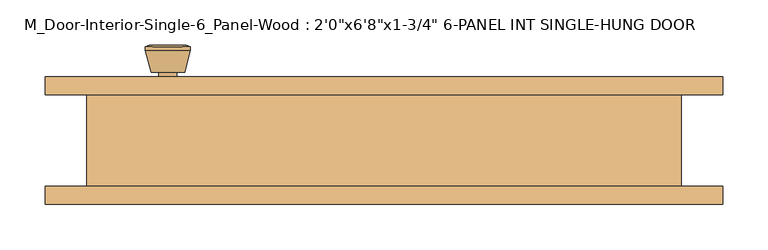
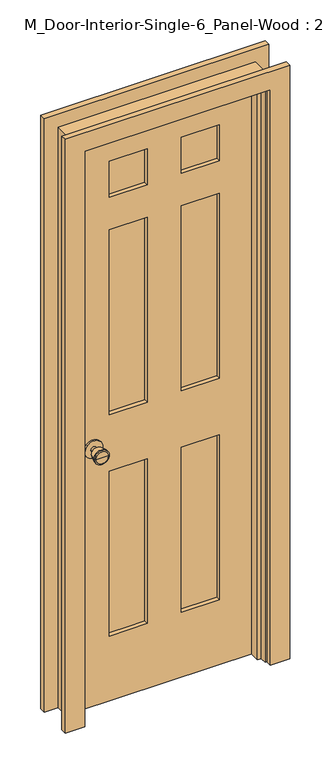
"""IFC4 building model written with IfcOpenShell, lengths in millimetres: door geometry."""

from ifc_helpers import new_model, si_unit, point, frame, frame_2d, origin, place, context, project, spatial, polyline, circle_curve, trimmed, segment, composite_curve, outline, extrude, faceted_brep, source, transform, mapped, element, save
from ifc_brep_helpers import plane_surface, cylinder_surface, revolved_surface, advanced_brep


def door_8ef89e6c(model_context):
    return source(origin(), model_context, "Body", "SolidModel", [
        advanced_brep(
        [(-239.8, -2.825, 914.4), (-229.8, -2.825, 914.4), (-249.8, -2.825, 914.4), (-219.3241324, -51.825, 914.4), (-239.8, -51.825, 914.4), (-260.2758676, -51.825, 914.4), (-214.8, -49.9971319, 914.4), (-264.8, -49.9971319, 914.4), (-214.8, -46.5334537, 914.4), (-264.8, -46.5334537, 914.4), (-221.163764, -21.825, 914.4), (-258.436236, -21.825, 914.4), (-229.8, -21.825, 914.4), (-249.8, -21.825, 914.4)],
        [
            (0, 1),
            (1, 2, circle_curve(frame((-239.8, -2.825, 914.4), z_axis=(0.0, 1.0, 0.0), x_axis=(-1.0, 0.0, 0.0)), 10.0)),
            (2, 0),
            (2, 1, circle_curve(frame((-239.8, -2.825, 914.4), z_axis=(0.0, 1.0, 0.0), x_axis=(-1.0, 0.0, 0.0)), 10.0)),
            (3, 4),
            (4, 5),
            (5, 3, circle_curve(frame((-239.8, -51.825, 914.4), z_axis=(0.0, -1.0, 0.0), x_axis=(-1.0, 0.0, 0.0)), 20.4758676)),
            (3, 5, circle_curve(frame((-239.8, -51.825, 914.4), z_axis=(0.0, -1.0, 0.0), x_axis=(-1.0, 0.0, 0.0)), 20.4758676)),
            (6, 3),
            (5, 7),
            (7, 6, circle_curve(frame((-239.8, -49.9971319, 914.4), z_axis=(0.0, -1.0, 0.0), x_axis=(-1.0, 0.0, 0.0)), 25.0)),
            (6, 7, circle_curve(frame((-239.8, -49.9971319, 914.4), z_axis=(0.0, -1.0, 0.0), x_axis=(-1.0, 0.0, 0.0)), 25.0)),
            (8, 6),
            (7, 9),
            (9, 8, circle_curve(frame((-239.8, -46.5334537, 914.4), z_axis=(0.0, -1.0, 0.0), x_axis=(-1.0, 0.0, 0.0)), 25.0)),
            (8, 9, circle_curve(frame((-239.8, -46.5334537, 914.4), z_axis=(0.0, -1.0, 0.0), x_axis=(-1.0, 0.0, 0.0)), 25.0)),
            (10, 8),
            (9, 11),
            (11, 10, circle_curve(frame((-239.8, -21.825, 914.4), z_axis=(0.0, -1.0, 0.0), x_axis=(-1.0, 0.0, 0.0)), 18.636236)),
            (10, 11, circle_curve(frame((-239.8, -21.825, 914.4), z_axis=(0.0, -1.0, 0.0), x_axis=(-1.0, 0.0, 0.0)), 18.636236)),
            (12, 10),
            (11, 13),
            (13, 12, circle_curve(frame((-239.8, -21.825, 914.4), z_axis=(0.0, -1.0, 0.0), x_axis=(-1.0, 0.0, 0.0)), 10.0)),
            (12, 13, circle_curve(frame((-239.8, -21.825, 914.4), z_axis=(0.0, -1.0, 0.0), x_axis=(-1.0, 0.0, 0.0)), 10.0)),
            (1, 12),
            (13, 2),
        ],
        [
            plane_surface(frame((-239.8, -2.825, 914.4), z_axis=(0.0, 1.0, 0.0), x_axis=(-1.0, 0.0, 0.0))),
            plane_surface(frame((-239.8, -51.825, 914.4), z_axis=(0.0, -1.0, 0.0), x_axis=(-1.0, 0.0, 0.0))),
            revolved_surface(polyline([(-260.2758676, -51.825, 914.4), (-264.8, -49.9971319, 914.4)]), (-239.8, -2.825, 914.4), (0.0, 1.0, 0.0)),
            cylinder_surface(frame((-239.8, -2.825, 914.4), z_axis=(0.0, 1.0, 0.0), x_axis=(-1.0, 0.0, 0.0)), 25.0),
            revolved_surface(polyline([(-264.8, -46.5334537, 914.4), (-258.436236, -21.825, 914.4)]), (-239.8, -2.825, 914.4), (0.0, 1.0, 0.0)),
            plane_surface(frame((-239.8, -21.825, 914.4), z_axis=(0.0, 1.0, 0.0), x_axis=(-1.0, 0.0, 0.0))),
            cylinder_surface(frame((-239.8, -2.825, 914.4), z_axis=(0.0, 1.0, 0.0), x_axis=(-1.0, 0.0, 0.0)), 10.0),
        ],
        [
            (0, [[1, 2, 3]]),
            (0, [[-3, 4, -1]]),
            (1, [[5, 6, 7]]),
            (1, [[-6, -5, 8]]),
            (2, [[9, -7, 10, 11]]),
            (2, [[-10, -8, -9, 12]]),
            (3, [[13, -11, 14, 15]]),
            (3, [[-14, -12, -13, 16]]),
            (4, [[17, -15, 18, 19]]),
            (4, [[-18, -16, -17, 20]]),
            (5, [[21, -19, 22, 23]]),
            (5, [[-22, -20, -21, 24]]),
            (6, [[25, -23, 26, -2]]),
            (6, [[-26, -24, -25, -4]]),
        ],
    ),
        extrude(outline(composite_curve([segment(trimmed(circle_curve(frame_2d((914.4, -239.8)), 30.0), [point((914.4, -269.8))], [point((914.4, -209.8))], False, "CARTESIAN"), True, "CONTINUOUS"), segment(trimmed(circle_curve(frame_2d((914.4, -239.8)), 30.0), [point((914.4, -209.8))], [point((914.4, -269.8))], False, "CARTESIAN"), True, "CONTINUOUS")], self_intersect=False)), frame((0.0, -2.825, 0.0), z_axis=(0.0, 1.0, 0.0), x_axis=(0.0, 0.0, 1.0)), (0.0, 0.0, 1.0), 6.0),
        advanced_brep(
        [(-239.8, 53.625, 914.4), (-249.8, 53.625, 914.4), (-229.8, 53.625, 914.4), (-219.3241324, 102.625, 914.4), (-260.2758676, 102.625, 914.4), (-239.8, 102.625, 914.4), (-214.8, 100.7971319, 914.4), (-264.8, 100.7971319, 914.4), (-214.8, 97.3334537, 914.4), (-264.8, 97.3334537, 914.4), (-221.163764, 72.625, 914.4), (-258.436236, 72.625, 914.4), (-229.8, 72.625, 914.4), (-249.8, 72.625, 914.4)],
        [
            (0, 1),
            (1, 2, circle_curve(frame((-239.8, 53.625, 914.4), z_axis=(0.0, -1.0, 0.0), x_axis=(-1.0, 0.0, 0.0)), 10.0)),
            (2, 0),
            (2, 1, circle_curve(frame((-239.8, 53.625, 914.4), z_axis=(0.0, -1.0, 0.0), x_axis=(-1.0, 0.0, 0.0)), 10.0)),
            (3, 4, circle_curve(frame((-239.8, 102.625, 914.4), z_axis=(0.0, 1.0, 0.0), x_axis=(-1.0, 0.0, 0.0)), 20.4758676)),
            (4, 5),
            (5, 3),
            (4, 3, circle_curve(frame((-239.8, 102.625, 914.4), z_axis=(0.0, 1.0, 0.0), x_axis=(-1.0, 0.0, 0.0)), 20.4758676)),
            (6, 7, circle_curve(frame((-239.8, 100.7971319, 914.4), z_axis=(0.0, 1.0, 0.0), x_axis=(-1.0, 0.0, 0.0)), 25.0)),
            (7, 4),
            (3, 6),
            (7, 6, circle_curve(frame((-239.8, 100.7971319, 914.4), z_axis=(0.0, 1.0, 0.0), x_axis=(-1.0, 0.0, 0.0)), 25.0)),
            (8, 9, circle_curve(frame((-239.8, 97.3334537, 914.4), z_axis=(0.0, 1.0, 0.0), x_axis=(-1.0, 0.0, 0.0)), 25.0)),
            (9, 7),
            (6, 8),
            (9, 8, circle_curve(frame((-239.8, 97.3334537, 914.4), z_axis=(0.0, 1.0, 0.0), x_axis=(-1.0, 0.0, 0.0)), 25.0)),
            (10, 11, circle_curve(frame((-239.8, 72.625, 914.4), z_axis=(0.0, 1.0, 0.0), x_axis=(-1.0, 0.0, 0.0)), 18.636236)),
            (11, 9),
            (8, 10),
            (11, 10, circle_curve(frame((-239.8, 72.625, 914.4), z_axis=(0.0, 1.0, 0.0), x_axis=(-1.0, 0.0, 0.0)), 18.636236)),
            (12, 13, circle_curve(frame((-239.8, 72.625, 914.4), z_axis=(0.0, 1.0, 0.0), x_axis=(-1.0, 0.0, 0.0)), 10.0)),
            (13, 11),
            (10, 12),
            (13, 12, circle_curve(frame((-239.8, 72.625, 914.4), z_axis=(0.0, 1.0, 0.0), x_axis=(-1.0, 0.0, 0.0)), 10.0)),
            (1, 13),
            (12, 2),
        ],
        [
            plane_surface(frame((-239.8, 53.625, 914.4), z_axis=(0.0, -1.0, 0.0), x_axis=(-1.0, 0.0, 0.0))),
            plane_surface(frame((-239.8, 102.625, 914.4), z_axis=(0.0, 1.0, 0.0), x_axis=(-1.0, 0.0, 0.0))),
            revolved_surface(polyline([(-260.2758676, 102.625, 914.4), (-264.8, 100.7971319, 914.4)]), (-239.8, 53.625, 914.4), (0.0, -1.0, 0.0)),
            cylinder_surface(frame((-239.8, 53.625, 914.4), z_axis=(0.0, -1.0, 0.0), x_axis=(-1.0, 0.0, 0.0)), 25.0),
            revolved_surface(polyline([(-264.8, 97.3334537, 914.4), (-258.436236, 72.625, 914.4)]), (-239.8, 53.625, 914.4), (0.0, -1.0, 0.0)),
            plane_surface(frame((-239.8, 72.625, 914.4), z_axis=(0.0, -1.0, 0.0), x_axis=(-1.0, 0.0, 0.0))),
            cylinder_surface(frame((-239.8, 53.625, 914.4), z_axis=(0.0, -1.0, 0.0), x_axis=(-1.0, 0.0, 0.0)), 10.0),
        ],
        [
            (0, [[1, 2, 3]]),
            (0, [[-3, 4, -1]]),
            (1, [[5, 6, 7]]),
            (1, [[8, -7, -6]]),
            (2, [[9, 10, -5, 11]]),
            (2, [[12, -11, -8, -10]]),
            (3, [[13, 14, -9, 15]]),
            (3, [[16, -15, -12, -14]]),
            (4, [[17, 18, -13, 19]]),
            (4, [[20, -19, -16, -18]]),
            (5, [[21, 22, -17, 23]]),
            (5, [[24, -23, -20, -22]]),
            (6, [[-2, 25, -21, 26]]),
            (6, [[-4, -26, -24, -25]]),
        ],
    ),
        extrude(outline(composite_curve([segment(trimmed(circle_curve(frame_2d((914.4, -239.8)), 30.0), [point((914.4, -269.8))], [point((914.4, -209.8))], False, "CARTESIAN"), True, "CONTINUOUS"), segment(trimmed(circle_curve(frame_2d((914.4, -239.8)), 30.0), [point((914.4, -209.8))], [point((914.4, -269.8))], False, "CARTESIAN"), True, "CONTINUOUS")], self_intersect=False)), frame((0.0, 47.625, 0.0), z_axis=(0.0, 1.0, 0.0), x_axis=(0.0, 0.0, 1.0)), (0.0, 0.0, 1.0), 6.0),
        extrude(outline(polyline([(184.8, 17.9916667), (57.5, 17.9916667), (57.5, 32.8083333), (184.8, 32.8083333), (184.8, 17.9916667)])), frame((0.0, 0.0, 1784.7), z_axis=(0.0, 0.0, 1.0), x_axis=(1.0, 0.0, 0.0)), (0.0, 0.0, 1.0), 127.3),
        extrude(outline(polyline([(184.8, 17.9916667), (57.5, 17.9916667), (57.5, 32.8083333), (184.8, 32.8083333), (184.8, 17.9916667)])), frame((0.0, 0.0, 1014.4), z_axis=(0.0, 0.0, 1.0), x_axis=(1.0, 0.0, 0.0)), (0.0, 0.0, 1.0), 655.3),
        extrude(outline(polyline([(-57.5, 17.9916667), (-184.8, 17.9916667), (-184.8, 32.8083333), (-57.5, 32.8083333), (-57.5, 17.9916667)])), frame((0.0, 0.0, 1014.4), z_axis=(0.0, 0.0, 1.0), x_axis=(1.0, 0.0, 0.0)), (0.0, 0.0, 1.0), 655.3),
        extrude(outline(polyline([(-57.5, 17.9916667), (-184.8, 17.9916667), (-184.8, 32.8083333), (-57.5, 32.8083333), (-57.5, 17.9916667)])), frame((0.0, 0.0, 1784.7), z_axis=(0.0, 0.0, 1.0), x_axis=(1.0, 0.0, 0.0)), (0.0, 0.0, 1.0), 127.3),
        extrude(outline(polyline([(184.8, 17.9916667), (57.5, 17.9916667), (57.5, 32.8083333), (184.8, 32.8083333), (184.8, 17.9916667)])), frame((0.0, 0.0, 230.0), z_axis=(0.0, 0.0, 1.0), x_axis=(1.0, 0.0, 0.0)), (0.0, 0.0, 1.0), 584.4),
        extrude(outline(polyline([(-57.5, 17.9916667), (-184.8, 17.9916667), (-184.8, 32.8083333), (-57.5, 32.8083333), (-57.5, 17.9916667)])), frame((0.0, 0.0, 230.0), z_axis=(0.0, 0.0, 1.0), x_axis=(1.0, 0.0, 0.0)), (0.0, 0.0, 1.0), 584.4),
        extrude(outline(polyline([(2032.0, -304.8), (0.0, -304.8), (0.0, 304.8), (2032.0, 304.8), (2032.0, -304.8)]), holes=[polyline([(1912.0, 57.5), (1912.0, 184.8), (1784.7, 184.8), (1784.7, 57.5), (1912.0, 57.5)]), polyline([(1669.7, 184.8), (1014.4, 184.8), (1014.4, 57.5), (1669.7, 57.5), (1669.7, 184.8)]), polyline([(1014.4, -57.5), (1014.4, -184.8), (1669.7, -184.8), (1669.7, -57.5), (1014.4, -57.5)]), polyline([(1784.7, -184.8), (1912.0, -184.8), (1912.0, -57.5), (1784.7, -57.5), (1784.7, -184.8)]), polyline([(814.4, 57.5), (814.4, 184.8), (230.0, 184.8), (230.0, 57.5), (814.4, 57.5)]), polyline([(230.0, -57.5), (230.0, -184.8), (814.4, -184.8), (814.4, -57.5), (230.0, -57.5)])]), frame((0.0, 3.175, 0.0), z_axis=(0.0, 1.0, 0.0), x_axis=(0.0, 0.0, 1.0)), (0.0, 0.0, 1.0), 44.45),
        faceted_brep([(329.8, 47.625, 0.0), (329.8, -53.975, 0.0), (304.8, -53.975, 0.0), (304.8, -31.75, 0.0), (292.1, -31.75, 0.0), (292.1, 3.175, 0.0), (304.8, 3.175, 0.0), (304.8, 47.625, 0.0), (329.8, 47.625, 2057.0), (329.8, -53.975, 2057.0), (-329.8, -53.975, 2057.0), (-329.8, -53.975, 0.0), (-304.8, -53.975, 0.0), (-304.8, -53.975, 2032.0), (304.8, -53.975, 2032.0), (304.8, -31.75, 2032.0), (-304.8, -31.75, 2032.0), (-304.8, -31.75, 0.0), (-292.1, -31.75, 0.0), (-292.1, -31.75, 2019.3), (292.1, -31.75, 2019.3), (292.1, 3.175, 2019.3), (-292.1, 3.175, 2019.3), (-292.1, 3.175, 0.0), (-304.8, 3.175, 0.0), (-304.8, 3.175, 2032.0), (304.8, 3.175, 2032.0), (304.8, 47.625, 2032.0), (-304.8, 47.625, 2032.0), (-304.8, 47.625, 0.0), (-329.8, 47.625, 0.0), (-329.8, 47.625, 2057.0)], [[[0, 1, 2, 3, 4, 5, 6, 7]], [[1, 0, 8, 9]], [[2, 1, 9, 10, 11, 12, 13, 14]], [[3, 2, 14, 15]], [[4, 3, 15, 16, 17, 18, 19, 20]], [[5, 4, 20, 21]], [[6, 5, 21, 22, 23, 24, 25, 26]], [[7, 6, 26, 27]], [[0, 7, 27, 28, 29, 30, 31, 8]], [[9, 8, 31, 10]], [[15, 14, 13, 16]], [[21, 20, 19, 22]], [[27, 26, 25, 28]], [[30, 29, 24, 23, 18, 17, 12, 11]], [[10, 31, 30, 11]], [[16, 13, 12, 17]], [[22, 19, 18, 23]], [[28, 25, 24, 29]]]),
        extrude(outline(polyline([(0.0, 311.15), (0.0, 376.15), (2103.35, 376.15), (2103.35, -376.15), (0.0, -376.15), (0.0, -311.15), (2038.35, -311.15), (2038.35, 311.15), (0.0, 311.15)])), frame((0.0, -73.975, 0.0), z_axis=(0.0, 1.0, 0.0), x_axis=(0.0, 0.0, 1.0)), (0.0, 0.0, 1.0), 20.0),
        extrude(outline(polyline([(0.0, 311.15), (0.0, 376.15), (2103.35, 376.15), (2103.35, -376.15), (0.0, -376.15), (0.0, -311.15), (2038.35, -311.15), (2038.35, 311.15), (0.0, 311.15)])), frame((0.0, 47.625, 0.0), z_axis=(0.0, 1.0, 0.0), x_axis=(0.0, 0.0, 1.0)), (0.0, 0.0, 1.0), 20.0),
    ])


if __name__ == "__main__":
    model = new_model("IFC4")
    model_context = context("Model", 3, world=origin())
    ifc_project = project(units=[si_unit("LENGTHUNIT", "METRE", prefix="MILLI")], contexts=[model_context])
    site = spatial("IfcSite", under=ifc_project)
    building = spatial("IfcBuilding", under=site)
    placement = place(None, origin())
    door_shape = door_8ef89e6c(model_context)
    element("IfcDoor", 1, ObjectType="M_Door-Interior-Single-6_Panel-Wood : 2'0\"x6'8\"x1-3/4\" 6-PANEL INT SINGLE-HUNG DOOR", at=placement, inside=building, context=model_context, shape_type="MappedRepresentation", body=[
        mapped(door_shape, transform((0.0, 0.0, 0.0), x_axis=(1.0, 0.0, 0.0), y_axis=(0.0, 1.0, 0.0), z_axis=(0.0, 0.0, 1.0))),
    ])
    save(model, "model.ifc")

# Revit data of these elements
# Type "M_Door-Interior-Single-6_Panel-Wood : 2'0\"x6'8\"x1-3/4\" 6-PANEL INT SINGLE-HUNG DOOR"
#   Type Mark = "10"
#   Assembly Code = "C1020300"
#   Analytic Construction = "Wooden"
#   Top Rail = 0' - 4.72441"
#   Top Panel = 0' - 5.01181"
#   Thickness = 0' - 1 3/4"
#   Thermal Resistance (R) = 2.5876 (h·ft²·°F)/BTU
#   Swing Angle [instance default] = 90.00°
#   Stiles = 0' - 4.72441"
#   Rough Width = 2' - 1.9685"
#   Rough Height = 6' - 8.98425"
#   Mullion = 0' - 4.52756"
#   Lock Rail = 0' - 7.87402"
#   Intermediate Rail = 0' - 4.52756"
#   Height = 6' - 8"
#   Width = 2' - 0"
#   Heat Transfer Coefficient (U) = 0.3865 BTU/(h·ft²·°F)
#   Bottom Rail = 0' - 9.05512"
#   Trim Material = Cherry
#   Panel Material = Cherry
#   Frame Material = Cherry
#   Door Handle Material = Aluminum
#   Visual Light Transmittance = 0
#   Solar Heat Gain Coefficient = 0
#   Wall Closure = (empty or 0)
#   Function = (empty or 0)
# Element 1 (IfcDoor, "M_Door-Interior-Single-6_Panel-Wood : 2'0\"x6'8\"x1-3/4\" 6-PANEL INT SINGLE-HUNG DOOR")
#   Materials on its faces: "Cherry", "Aluminum"
# Materials
#   "Cherry": class "Wood", colour RGB 226 177 128, transparency 0, Description = "Prunus Serotina", Cost = 0
#   "Aluminum": class "Metal", colour RGB 244 244 244, transparency 0, Description = "Aluminum 6061", Cost = 0
